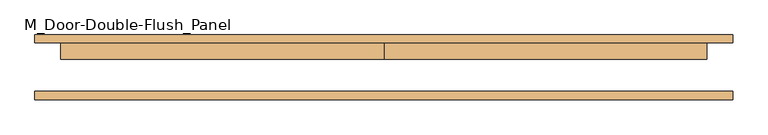
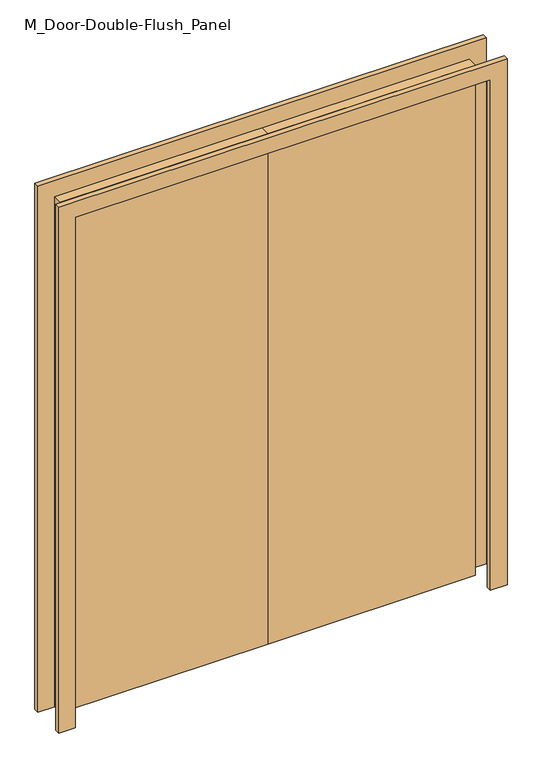
"""IFC4 building model written with IfcOpenShell, lengths in millimetres: door geometry, M_Door-Double-Flush_Panel : 2200 x 2600mm DAPC."""

from ifc_helpers import new_model, si_unit, frame, origin, origin_with_axes, place, context, project, spatial, polyline, outline, extrude, source, transform, mapped, element, save


def m_door_double_flush_panel_3c273409(model_context):
    return source(origin(), model_context, "Body", "SweptSolid", [
        extrude(outline(polyline([(2600.0, -1000.0), (2600.0, 1000.0), (0.0, 1000.0), (0.0, 1080.0), (2680.0, 1080.0), (2680.0, -1080.0), (0.0, -1080.0), (0.0, -1000.0), (2600.0, -1000.0)])), frame((0.0, 75.0, 0.0), z_axis=(0.0, 1.0, 0.0), x_axis=(0.0, 0.0, 1.0)), (0.0, 0.0, 1.0), 25.0),
        extrude(outline(polyline([(2600.0, -1000.0), (2600.0, 1000.0), (0.0, 1000.0), (0.0, 1080.0), (2680.0, 1080.0), (2680.0, -1080.0), (0.0, -1080.0), (0.0, -1000.0), (2600.0, -1000.0)])), frame((0.0, -100.0, 0.0), z_axis=(0.0, 1.0, 0.0), x_axis=(0.0, 0.0, 1.0)), (0.0, 0.0, 1.0), 25.0),
        extrude(outline(polyline([(-1000.0, 75.0), (0.0, 75.0), (0.0, 25.0), (-1000.0, 25.0), (-1000.0, 75.0)])), origin_with_axes(), (0.0, 0.0, 1.0), 2600.0),
        extrude(outline(polyline([(0.0, 75.0), (1000.0, 75.0), (1000.0, 25.0), (0.0, 25.0), (0.0, 75.0)])), origin_with_axes(), (0.0, 0.0, 1.0), 2600.0),
    ])


if __name__ == "__main__":
    model = new_model("IFC4")
    model_context = context("Model", 3, world=origin())
    ifc_project = project(units=[si_unit("LENGTHUNIT", "METRE", prefix="MILLI")], contexts=[model_context])
    site = spatial("IfcSite", under=ifc_project)
    building = spatial("IfcBuilding", under=site)
    placement = place(None, origin())
    m_door_double_flush_panel_shape = m_door_double_flush_panel_3c273409(model_context)
    element("IfcDoor", 1, ObjectType="M_Door-Double-Flush_Panel : 2200 x 2600mm DAPC", at=placement, inside=building, context=model_context, shape_type="MappedRepresentation", body=[
        mapped(m_door_double_flush_panel_shape, transform((0.0, 0.0, 0.0), x_axis=(1.0, 0.0, 0.0), y_axis=(0.0, 1.0, 0.0), z_axis=(0.0, 0.0, 1.0))),
    ])
    save(model, "model.ifc")

# Revit data of these elements
# Type "M_Door-Double-Flush_Panel : 2200 x 2600mm DAPC"
#   Type Mark = "47"
#   Construction Type Id = "DOOR"
#   Analytic Construction = "Wooden"
#   Thickness = 0.05 m
#   Thermal Resistance (R) = 0.455703 (m²·K)/W
#   Swing Angle [instance default] = 90.00°
#   Panel Width = 1.00 m
#   Heat Transfer Coefficient (U) = 2.19465 W/(m²·K)
#   Height = 2.60 m
#   Trim Projection Ext = 0.025 m
#   Trim Projection Int = 0.025 m
#   Trim Width = 0.08 m
#   Width = 2.00 m
#   Define Thermal Properties by = 1
#   Panel Material = Wood - Birch - Solid Stained Light Low Gloss
#   Trim Material = Paint - Sienna
#   Visual Light Transmittance = 0
#   Solar Heat Gain Coefficient = 0
#   Function = (empty or 0)
#   Wall Closure = (empty or 0)
# Element 1 (IfcDoor, "M_Door-Double-Flush_Panel : 2200 x 2600mm DAPC")
#   Materials on its faces: "Paint - Sienna", "Wood - Birch - Solid Stained Light Low Gloss"
# Materials
#   "Wood - Birch - Solid Stained Light Low Gloss": class "Wood", colour RGB 210 159 95, transparency 0, Cost = 0
#   "Paint - Sienna": class "Miscellaneous", colour RGB 118 70 51, transparency 0, Cost = 0
